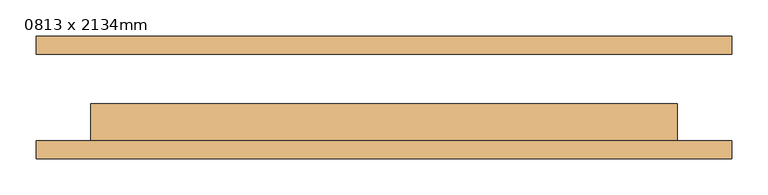
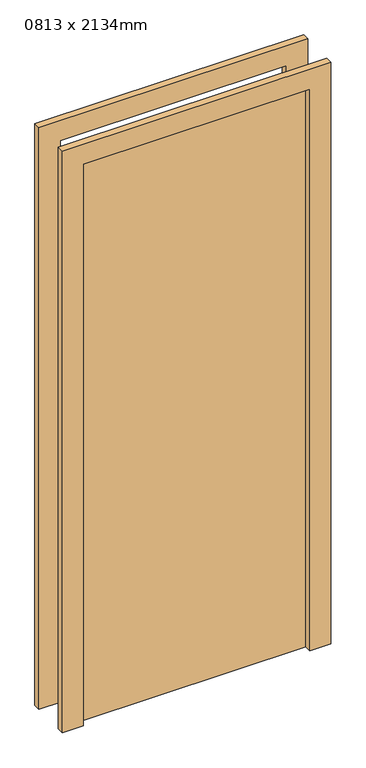
"""IFC4 building model written with IfcOpenShell, lengths in millimetres: door geometry, M_Folha única : 0813 x 2134mm."""

import ifcopenshell
import ifcopenshell.guid

model = None  # the IFC model being written
_history = None  # IfcOwnerHistory: only IFC2X3 demands one
_inside = {}  # id of a spatial element -> (the spatial element, [elements in it])
_under = {}  # id of a project, library or spatial element -> (it, [spatial elements below it])
_declared = {}  # id of a project -> (the project, [libraries it declares])
_typed = {}  # id of a type object -> (the type object, [elements of that type])
_made_of = {}  # id of a material, layer set ... -> (it, [elements and type objects made of it])


def new_model(schema):
    """Start an empty IFC model of exactly this schema.

    Asked for "IFC4X3", IfcOpenShell would pick the latest addendum, in which some entities
    have other attributes; the version numbers below select the first issue.
    IFC2X3 requires an IfcOwnerHistory on every rooted entity: one is made here for all.
    """
    global model, _history
    if schema == "IFC4X3":
        model = ifcopenshell.file(schema_version=(4, 3, 0, 0))
    else:
        model = ifcopenshell.file(schema=schema)
    _inside.clear()
    _under.clear()
    _declared.clear()
    _typed.clear()
    _made_of.clear()
    _history = None
    if model.schema == "IFC2X3":
        org = make("IfcOrganization", Name="unknown")
        user = make(
            "IfcPersonAndOrganization",
            ThePerson=make("IfcPerson", FamilyName="unknown"),
            TheOrganization=org,
        )
        app = make(
            "IfcApplication",
            ApplicationDeveloper=org,
            Version="unknown",
            ApplicationFullName="unknown",
            ApplicationIdentifier="unknown",
        )
        _history = make(
            "IfcOwnerHistory",
            OwningUser=user,
            OwningApplication=app,
            ChangeAction="ADDED",
            CreationDate=0,
        )
    return model


def make(cls, **values):
    """One entity of the class cls with the attributes given. An attribute that is None is left unset."""
    return model.create_entity(
        cls, **{name: value for name, value in values.items() if value is not None}
    )


def rooted(cls, **values):
    """An entity with a GlobalId (a new one), such as an element, a storey or a relation."""
    return make(cls, GlobalId=ifcopenshell.guid.new(), OwnerHistory=_history, **values)


def si_unit(unit_type, name, prefix=None):
    """IfcSIUnit, for example si_unit("LENGTHUNIT", "METRE", prefix="MILLI")."""
    return make("IfcSIUnit", UnitType=unit_type, Prefix=prefix, Name=name)


def assignment(units):
    """IfcUnitAssignment: the units of a project."""
    return None if units is None else make("IfcUnitAssignment", Units=units)


def point(xyz):
    """IfcCartesianPoint."""
    return None if xyz is None else make("IfcCartesianPoint", Coordinates=xyz)


def direction(xyz):
    """IfcDirection."""
    return None if xyz is None else make("IfcDirection", DirectionRatios=xyz)


def frame(location, z_axis=None, x_axis=None):
    """IfcAxis2Placement3D, a coordinate frame: its origin and axes. An axis left out is left unset."""
    return make(
        "IfcAxis2Placement3D",
        Location=point(location),
        Axis=direction(z_axis),
        RefDirection=direction(x_axis),
    )


def origin():
    """The frame at (0, 0, 0) with its axes left unset."""
    return frame((0.0, 0.0, 0.0))


def origin_with_axes():
    """The frame at (0, 0, 0) with the z axis (0, 0, 1) and the x axis (1, 0, 0) written out."""
    return frame((0.0, 0.0, 0.0), z_axis=(0.0, 0.0, 1.0), x_axis=(1.0, 0.0, 0.0))


def place(relative_to, where):
    """IfcLocalPlacement: puts the frame where relative to a parent placement (None: the world)."""
    return make(
        "IfcLocalPlacement", PlacementRelTo=relative_to, RelativePlacement=where
    )


def context(
    kind, dimensions, precision=None, world=None, true_north=None, identifier=None
):
    """IfcGeometricRepresentationContext, for example the 3D "Model" context."""
    return make(
        "IfcGeometricRepresentationContext",
        ContextIdentifier=identifier,
        ContextType=kind,
        CoordinateSpaceDimension=dimensions,
        Precision=precision,
        WorldCoordinateSystem=world,
        TrueNorth=true_north,
    )


def project(units=None, contexts=None):
    """IfcProject with its units and contexts."""
    return rooted(
        "IfcProject",
        Name="project",
        RepresentationContexts=contexts,
        UnitsInContext=assignment(units),
    )


def spatial(cls, under=None, at=None, **own):
    """A site, building, storey or space (cls), placed at a placement, below another one or the project."""
    s = rooted(cls, ObjectPlacement=at, **own)
    if under is not None:
        _under.setdefault(under.id(), (under, []))[1].append(s)
    return s


def polyline(points):
    """IfcPolyline through the points."""
    return make("IfcPolyline", Points=[point(p) for p in points])


def outline(outer, holes=None, kind="AREA"):
    """IfcArbitraryClosedProfileDef: a profile drawn as a closed curve; with holes, ...WithVoids."""
    if holes is None:
        return make("IfcArbitraryClosedProfileDef", ProfileType=kind, OuterCurve=outer)
    return make(
        "IfcArbitraryProfileDefWithVoids",
        ProfileType=kind,
        OuterCurve=outer,
        InnerCurves=holes,
    )


def extrude(swept, where, along, depth):
    """IfcExtrudedAreaSolid: the profile swept, set in the frame where, extruded along a direction by depth."""
    return make(
        "IfcExtrudedAreaSolid",
        SweptArea=swept,
        Position=where,
        ExtrudedDirection=direction(along),
        Depth=depth,
    )


def shape(context_of_items, identifier, shape_type, items):
    """IfcShapeRepresentation: the items that make up one representation, for example the "Body"."""
    return make(
        "IfcShapeRepresentation",
        ContextOfItems=context_of_items,
        RepresentationIdentifier=identifier,
        RepresentationType=shape_type,
        Items=items,
    )


def source(mapping_origin, context_of_items, identifier, shape_type, items):
    """IfcRepresentationMap: a shape defined once, which mapped items show again and again."""
    return make(
        "IfcRepresentationMap",
        MappingOrigin=mapping_origin,
        MappedRepresentation=shape(context_of_items, identifier, shape_type, items),
    )


def transform(
    local_origin,
    x_axis=None,
    y_axis=None,
    z_axis=None,
    scale=None,
    scale2=None,
    scale3=None,
    uniform=True,
):
    """IfcCartesianTransformationOperator3D, or its non-uniform kind. x_axis, y_axis, z_axis: its Axis1, 2, 3."""
    if uniform:
        return make(
            "IfcCartesianTransformationOperator3D",
            Axis1=direction(x_axis),
            Axis2=direction(y_axis),
            LocalOrigin=point(local_origin),
            Scale=scale,
            Axis3=direction(z_axis),
        )
    return make(
        "IfcCartesianTransformationOperator3DnonUniform",
        Axis1=direction(x_axis),
        Axis2=direction(y_axis),
        LocalOrigin=point(local_origin),
        Scale=scale,
        Axis3=direction(z_axis),
        Scale2=scale2,
        Scale3=scale3,
    )


def mapped(mapping_source, mapping_target):
    """IfcMappedItem: shows the shape of a source again, moved by a transform."""
    return make(
        "IfcMappedItem", MappingSource=mapping_source, MappingTarget=mapping_target
    )


def made_of(thing, what):
    """Note that an element or type object is made of a material, layer set ...; save() writes the relation."""
    if what is not None:
        _made_of.setdefault(what.id(), (what, []))[1].append(thing)
    return thing


def element(
    cls,
    number,
    at=None,
    inside=None,
    cuts=None,
    type_object=None,
    material=None,
    context=None,
    identifier="Body",
    shape_type=None,
    held_by="IfcProductDefinitionShape",
    body=None,
    shapes=None,
    **own,
):
    """One element of the class cls, such as IfcWall. Its Tag is "e" and its number.

    at: its placement. inside: the storey or other place that contains it. cuts: it is an
    opening in that element (IfcRelVoidsElement). A single representation is given by context,
    identifier, shape_type and body (its items); several are given by shapes. held_by: the class
    of the entity that holds the representations. save() writes the other relations.
    """
    e = rooted(cls, Tag="e%d" % number, ObjectPlacement=at, **own)
    if body is not None:
        shapes = [shape(context, identifier, shape_type, body)]
    if shapes is not None:
        e.Representation = make(held_by, Representations=shapes)
    if inside is not None:
        _inside.setdefault(inside.id(), (inside, []))[1].append(e)
    if cuts is not None:
        rooted(
            "IfcRelVoidsElement", RelatingBuildingElement=cuts, RelatedOpeningElement=e
        )
    if type_object is not None:
        _typed.setdefault(type_object.id(), (type_object, []))[1].append(e)
    return made_of(e, material)


def aggregate(whole, parts):
    """IfcRelAggregates: a whole, such as a stair, and the parts it consists of."""
    return rooted("IfcRelAggregates", RelatingObject=whole, RelatedObjects=parts)


def save(model, path):
    """Write the relations noted so far, then the file.

    IfcRelAggregates (storeys below a building ...), IfcRelContainedInSpatialStructure (elements
    in a storey), IfcRelDefinesByType, IfcRelAssociatesMaterial and IfcRelDeclares: one each for
    every whole, place, type object, material and project.
    """
    for whole, parts in _under.values():
        aggregate(whole, parts)
    for where, things in _inside.values():
        rooted(
            "IfcRelContainedInSpatialStructure",
            RelatedElements=things,
            RelatingStructure=where,
        )
    for kind, things in _typed.values():
        rooted("IfcRelDefinesByType", RelatedObjects=things, RelatingType=kind)
    for what, things in _made_of.values():
        rooted("IfcRelAssociatesMaterial", RelatedObjects=things, RelatingMaterial=what)
    for by, libraries in _declared.values():
        rooted("IfcRelDeclares", RelatingContext=by, RelatedDefinitions=libraries)
    model.write(path)


def door_0813_x_2134mm_8eb04c96(model_context):
    return source(origin(), model_context, "Body", "SweptSolid", [
        extrude(outline(polyline([(2210.0, -482.5), (0.0, -482.5), (0.0, -406.5), (2134.0, -406.5), (2134.0, 406.5), (0.0, 406.5), (0.0, 482.5), (2210.0, 482.5), (2210.0, -482.5)])), frame((0.0, -85.0, 0.0), z_axis=(0.0, 1.0, 0.0), x_axis=(0.0, 0.0, 1.0)), (0.0, 0.0, 1.0), 25.0),
        extrude(outline(polyline([(2210.0, 482.5), (2210.0, -482.5), (0.0, -482.5), (0.0, -406.5), (2134.0, -406.5), (2134.0, 406.5), (0.0, 406.5), (0.0, 482.5), (2210.0, 482.5)])), frame((0.0, 60.0, 0.0), z_axis=(0.0, 1.0, 0.0), x_axis=(0.0, 0.0, 1.0)), (0.0, 0.0, 1.0), 25.0),
        extrude(outline(polyline([(406.5, -9.0), (406.5, -60.0), (-406.5, -60.0), (-406.5, -9.0), (406.5, -9.0)])), origin_with_axes(), (0.0, 0.0, 1.0), 2134.0),
    ])


if __name__ == "__main__":
    model = new_model("IFC4")
    model_context = context("Model", 3, world=origin())
    ifc_project = project(units=[si_unit("LENGTHUNIT", "METRE", prefix="MILLI")], contexts=[model_context])
    site = spatial("IfcSite", under=ifc_project)
    building = spatial("IfcBuilding", under=site)
    placement = place(None, origin())
    door_0813_x_2134mm_shape = door_0813_x_2134mm_8eb04c96(model_context)
    element("IfcDoor", 1, ObjectType="M_Folha única : 0813 x 2134mm", at=placement, inside=building, context=model_context, shape_type="MappedRepresentation", body=[
        mapped(door_0813_x_2134mm_shape, transform((0.0, 0.0, 0.0), x_axis=(1.0, 0.0, 0.0), y_axis=(0.0, 1.0, 0.0), z_axis=(0.0, 0.0, 1.0))),
    ])
    save(model, "model.ifc")

# Revit data of these elements
# Project information
#   Data de emissão do projeto = "Data de emissão"
#   Status do projeto = "Status do projeto"
#   Nome do cliente = "Proprietário"
#   Endereço do projeto = "Insira aqui o endereço"
#   Nome do projeto = "Nome do projeto"
#   Número do projeto = "0001"
# Type "M_Folha única : 0813 x 2134mm"
#   Type Mark = "24"
#   Construction Type Id = "MDOOR"
#   Analytic Construction = "Metal"
#   Thickness = 0.051 m
#   Thermal Resistance (R) = 0.270117 (m²·K)/W
#   Heat Transfer Coefficient (U) = 3.7021 W/(m²·K)
#   Height = 2.134 m
#   Projeção da apara externa = 0.025 m
#   Projeção da apara interna = 0.025 m
#   Largura da apara = 0.076 m
#   Width = 0.813 m
#   Define Thermal Properties by = 1
#   Material da porta = Porta - Painel
#   Material da moldura = Porta - Batente
#   Visual Light Transmittance = 0
#   Solar Heat Gain Coefficient = 0
#   Function = (empty or 0)
#   Wall Closure = (empty or 0)
# Element 1 (IfcDoor, "M_Folha única : 0813 x 2134mm")
#   Materials on its faces: "Porta - Batente", "Porta - Painel"
# Materials
#   "Porta - Painel": class "Madeira", colour RGB 210 159 95, transparency 0, Cost = 0
#   "Porta - Batente": class "Diversos", colour RGB 118 70 51, transparency 0, Cost = 0
